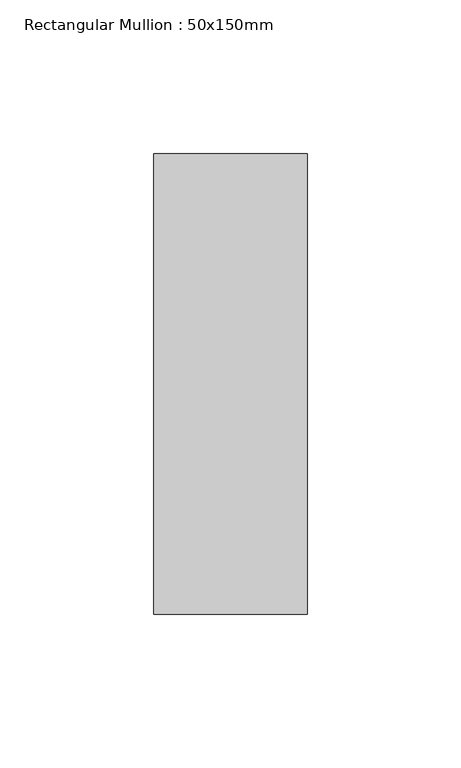
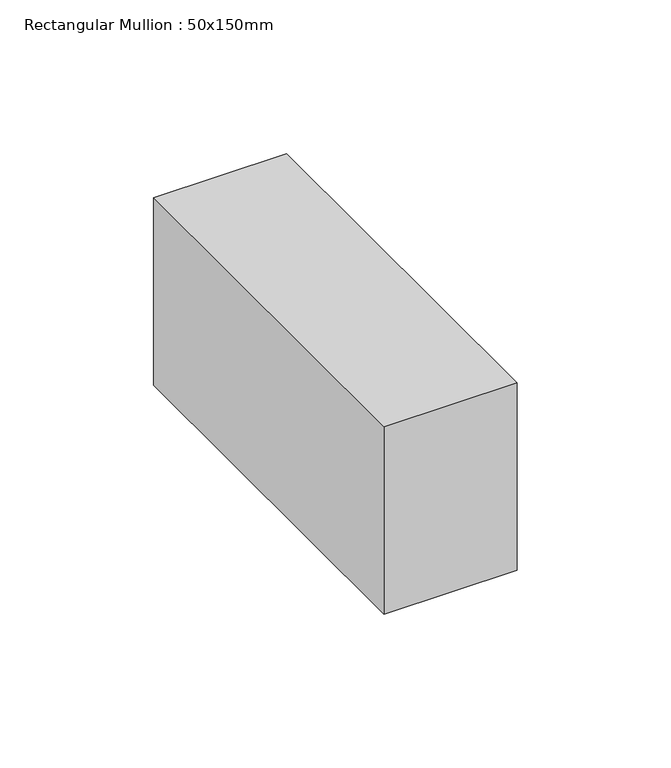
"""IFC4 building model written with IfcOpenShell, lengths in millimetres: member geometry, Rectangular Mullion : 50x150mm."""

from ifc_helpers import new_model, si_unit, frame, origin, place, context, project, spatial, polyline, outline, extrude, source, transform, mapped, element, save


def rectangular_mullion_50x150mm_6eefbde0(model_context):
    return source(origin(), model_context, "Body", "SweptSolid", [
        extrude(outline(polyline([(0.0, 75.0), (0.0, -75.0), (-50.0, -75.0), (-50.0, 75.0), (0.0, 75.0)])), frame((0.0, 0.0, -74.4185145), z_axis=(0.0, 0.0, 1.0), x_axis=(1.0, 0.0, 0.0)), (0.0, 0.0, 1.0), 74.4185145),
    ])


if __name__ == "__main__":
    model = new_model("IFC4")
    model_context = context("Model", 3, world=origin())
    ifc_project = project(units=[si_unit("LENGTHUNIT", "METRE", prefix="MILLI")], contexts=[model_context])
    site = spatial("IfcSite", under=ifc_project)
    building = spatial("IfcBuilding", under=site)
    placement = place(None, origin())
    rectangular_mullion_50x150mm_shape = rectangular_mullion_50x150mm_6eefbde0(model_context)
    element("IfcMember", 1, ObjectType="Rectangular Mullion : 50x150mm", at=placement, inside=building, context=model_context, shape_type="MappedRepresentation", body=[
        mapped(rectangular_mullion_50x150mm_shape, transform((0.0, 0.0, 0.0), x_axis=(1.0, 0.0, 0.0), y_axis=(0.0, 1.0, 0.0), z_axis=(0.0, 0.0, 1.0))),
    ])
    save(model, "model.ifc")

# Revit data of these elements
# Type "Rectangular Mullion : 50x150mm"
#   Keynote = "H11"
#   built-in parameter 1007304 = 0.492126 (stored number, unit not read)
#   built-in parameter 1007301 = 0.082021 (stored number, unit not read)
#   built-in parameter 1007300 = 0.082021 (stored number, unit not read)
# Element 1 (IfcMember, "Rectangular Mullion : 50x150mm")
#   Materials on its faces: "Aluminium"
# Materials
#   "Aluminium": class "Metal", colour RGB 247 247 247, transparency 0, Description = "Aluminium 6061", Cost = 0
